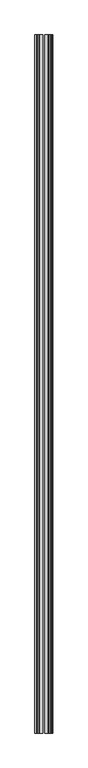
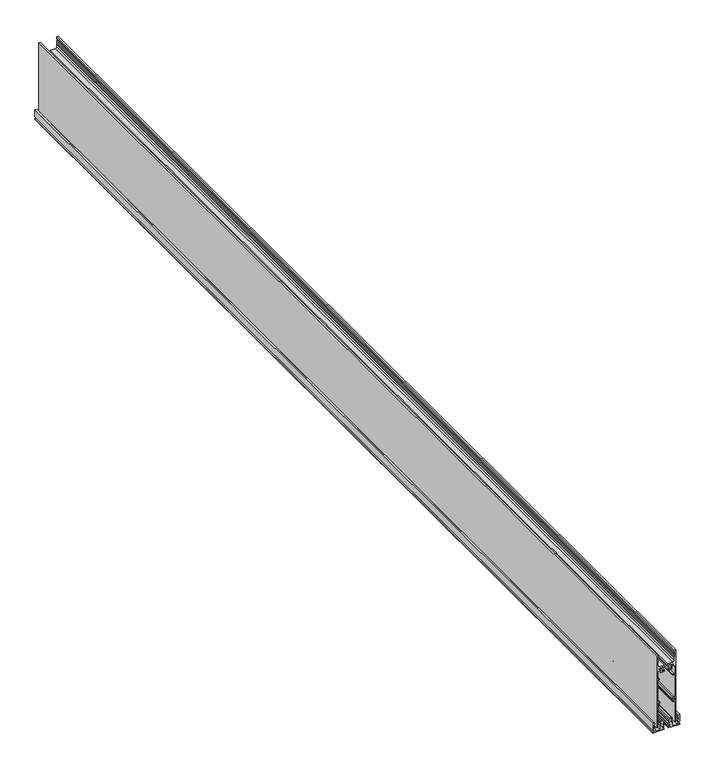
"""IFC4 building model written with IfcOpenShell, lengths in millimetres: proxy geometry, Structure002 653 : Structure002 653."""

from ifc_helpers import new_model, si_unit, frame, origin, place, context, project, spatial, polyline, outline, extrude, source, transform, mapped, element, save


def generic_models_8680b48e(model_context):
    return source(origin(), model_context, "Body", "SweptSolid", [
        extrude(outline(polyline([(37496.4365618, 7657.7930318), (37495.366697, 7656.7528175), (37493.1734209, 7656.7528175), (37493.1734209, 7657.8229747), (37494.7782571, 7657.8229747), (37494.7782571, 7659.1606712), (37486.7569596, 7659.1606712), (37486.7569596, 7657.8229747), (37488.3589123, 7657.8229747), (37488.3589123, 7656.7528175), (37485.0752597, 7656.7528175), (37483.4739937, 7655.8966918), (37479.1043438, 7655.8966918), (37479.1043438, 7646.8538638), (37488.3579135, 7646.8538638), (37488.3579135, 7645.7837066), (37486.7540761, 7645.7837066), (37486.7540761, 7644.4460101), (37494.7782571, 7644.4460101), (37494.7782571, 7645.7837066), (37493.1734209, 7645.7837066), (37493.1734209, 7646.8538638), (37495.366697, 7646.8538638), (37496.436721, 7645.7838398), (37496.436721, 7644.7135494), (37495.5512233, 7642.6415254), (37493.0931791, 7641.3693083), (37490.017243, 7641.3693083), (37490.017243, 7642.4394655), (37486.4063615, 7642.4394655), (37486.4063615, 7639.7636558), (37484.5340526, 7639.7636558), (37484.5340526, 7640.5671028), (37483.2789107, 7640.5671028), (37484.4508456, 7642.077477), (37484.4508456, 7643.199305), (37480.1257911, 7643.199305), (37479.7006783, 7643.9284483), (37479.2397502, 7643.1732751), (37479.2397502, 7641.7763334), (37480.6168771, 7641.7763334), (37480.6168771, 7640.2864915), (37479.8959721, 7639.724537), (37477.446, 7639.5315657), (37477.446, 7641.6449434), (37478.4679055, 7641.6449434), (37478.4679055, 7643.199305), (37477.446, 7643.199305), (37477.446, 7661.0334462), (37478.8903656, 7661.0334462), (37478.8903656, 7657.5554354), (37484.2874925, 7657.5554354), (37483.0336251, 7659.7088758), (37483.0336251, 7661.0334462), (37496.4365618, 7661.0334462), (37496.4365618, 7657.7930318)])), frame((0.0, -3747.9491938, 0.0), z_axis=(0.0, 1.0, 0.0), x_axis=(0.0, 0.0, 1.0)), (0.0, 0.0, 1.0), 2000.0),
        extrude(outline(polyline([(37483.0336251, 7610.0797736), (37483.0336251, 7611.404344), (37484.2874925, 7613.5577844), (37478.8903656, 7613.5577844), (37478.8903656, 7610.0797736), (37477.446, 7610.0797736), (37477.446, 7627.9139148), (37478.4679055, 7627.9139148), (37478.4679055, 7629.4682764), (37477.446, 7629.4682764), (37477.446, 7631.5816541), (37479.8959721, 7631.3886828), (37480.6168771, 7630.8267283), (37480.6168771, 7629.3368864), (37479.2397502, 7629.3368864), (37479.2397502, 7627.9399447), (37479.7006783, 7627.1847715), (37480.1257911, 7627.9139148), (37484.4508456, 7627.9139148), (37484.4508456, 7629.0357427), (37483.2789107, 7630.5461169), (37484.5340526, 7630.5461169), (37484.5340526, 7631.349564), (37486.4063615, 7631.349564), (37486.4063615, 7628.6737543), (37490.017243, 7628.6737543), (37490.017243, 7629.7439115), (37493.0931791, 7629.7439115), (37495.5512233, 7628.4716944), (37496.436721, 7626.3996703), (37496.436721, 7625.32938), (37495.366697, 7624.259356), (37493.1734209, 7624.259356), (37493.1734209, 7625.3295132), (37494.7782571, 7625.3295132), (37494.7782571, 7626.6672096), (37486.7540761, 7626.6672096), (37486.7540761, 7625.3295132), (37488.3579135, 7625.3295132), (37488.3579135, 7624.259356), (37479.1043438, 7624.259356), (37479.1043438, 7615.216528), (37483.4739937, 7615.216528), (37485.0752597, 7614.3604022), (37488.3589123, 7614.3604022), (37488.3589123, 7613.2902451), (37486.7569596, 7613.2902451), (37486.7569596, 7611.9525486), (37494.7782571, 7611.9525486), (37494.7782571, 7613.2902451), (37493.1734209, 7613.2902451), (37493.1734209, 7614.3604022), (37495.366697, 7614.3604022), (37496.4365618, 7613.320188), (37496.4365618, 7610.0797736), (37483.0336251, 7610.0797736)])), frame((0.0, -3747.9491938, 0.0), z_axis=(0.0, 1.0, 0.0), x_axis=(0.0, 0.0, 1.0)), (0.0, 0.0, 1.0), 2000.0),
        extrude(outline(polyline([(37604.2015618, 7622.5346434), (37606.7094313, 7620.0267738), (37611.5111794, 7620.0267738), (37613.3758754, 7620.5013448), (37616.0506024, 7619.6987269), (37616.0506024, 7620.5013448), (37618.7253294, 7619.6987269), (37618.7253294, 7620.5013448), (37621.4000564, 7619.6987269), (37621.4000564, 7620.5013448), (37624.0747835, 7619.6987269), (37624.0747835, 7620.5013448), (37626.7495105, 7620.5013448), (37626.7495105, 7617.5049047), (37485.4971771, 7617.5049047), (37485.4971771, 7620.019774), (37525.8320604, 7620.019774), (37525.8320604, 7622.9091984), (37527.4903911, 7622.9091984), (37527.4903911, 7621.9460569), (37529.4164343, 7620.0200138), (37532.9735815, 7620.0200138), (37532.9735815, 7621.8390412), (37531.2885035, 7621.8390412), (37531.2885035, 7623.444277), (37534.6319122, 7623.444277), (37534.6319122, 7620.019774), (37578.3369516, 7620.019774), (37578.3369516, 7622.9091984), (37579.9952823, 7622.9091984), (37579.9952823, 7620.019774), (37595.9502358, 7620.019774), (37595.9502358, 7620.9354673), (37597.8865057, 7622.2081155), (37599.3688896, 7621.4577733), (37600.7763445, 7621.4577733), (37601.7660928, 7623.391903), (37600.8580603, 7625.1625844), (37599.3688896, 7625.1625844), (37597.8866262, 7624.4666157), (37595.9502358, 7625.5845913), (37591.6838394, 7625.5845913), (37591.6838394, 7632.2730736), (37594.6795336, 7632.2730736), (37594.6795336, 7630.9353771), (37593.3421701, 7630.9353771), (37593.3421701, 7627.2433349), (37601.6873184, 7627.2433349), (37601.6873184, 7630.9353771), (37600.3499549, 7630.9353771), (37600.3499549, 7632.2730736), (37604.2015618, 7632.2730736), (37604.2015618, 7622.5346434)])), frame((0.0, -3747.9491938, 0.0), z_axis=(0.0, 1.0, 0.0), x_axis=(0.0, 0.0, 1.0)), (0.0, 0.0, 1.0), 2000.0),
        extrude(outline(polyline([(37600.3499549, 7638.8401462), (37600.3499549, 7640.1778427), (37601.6873184, 7640.1778427), (37601.6873184, 7643.8698849), (37593.3421701, 7643.8698849), (37593.3421701, 7640.1778427), (37594.6795336, 7640.1778427), (37594.6795336, 7638.8401462), (37591.6838394, 7638.8401462), (37591.6838394, 7645.5286285), (37595.9502358, 7645.5286285), (37597.8866262, 7646.646604), (37599.3688896, 7645.9506354), (37600.8580603, 7645.9506354), (37601.7660928, 7647.7213168), (37600.7763445, 7649.6554465), (37599.3688896, 7649.6554465), (37597.8865057, 7648.9051043), (37595.9502358, 7650.1777525), (37595.9502358, 7651.0934457), (37579.9952823, 7651.0934457), (37579.9952823, 7648.2040214), (37578.3369516, 7648.2040214), (37578.3369516, 7651.0934457), (37534.6319122, 7651.0934457), (37534.6319122, 7647.6689428), (37531.2885035, 7647.6689428), (37531.2885035, 7649.2741786), (37532.9735815, 7649.2741786), (37532.9735815, 7651.093206), (37529.4164343, 7651.093206), (37527.4903911, 7649.1671628), (37527.4903911, 7648.2040214), (37525.8320604, 7648.2040214), (37525.8320604, 7651.0934457), (37485.4971771, 7651.0934457), (37485.4971771, 7653.6083151), (37626.7495105, 7653.6083151), (37626.7495105, 7650.611875), (37624.0747835, 7650.611875), (37624.0747835, 7651.4144929), (37621.4000564, 7650.611875), (37621.4000564, 7651.4144929), (37618.7253294, 7650.611875), (37618.7253294, 7651.4144929), (37616.0506024, 7650.611875), (37616.0506024, 7651.4144929), (37613.3758754, 7650.611875), (37611.5111794, 7651.086446), (37606.7094313, 7651.086446), (37604.2015618, 7648.5785764), (37604.2015618, 7638.8401462), (37600.3499549, 7638.8401462)])), frame((0.0, -3747.9491938, 0.0), z_axis=(0.0, 1.0, 0.0), x_axis=(0.0, 0.0, 1.0)), (0.0, 0.0, 1.0), 2000.0),
    ])


if __name__ == "__main__":
    model = new_model("IFC4")
    model_context = context("Model", 3, world=origin())
    ifc_project = project(units=[si_unit("LENGTHUNIT", "METRE", prefix="MILLI")], contexts=[model_context])
    site = spatial("IfcSite", under=ifc_project)
    building = spatial("IfcBuilding", under=site)
    placement = place(None, origin())
    generic_models_shape = generic_models_8680b48e(model_context)
    element("IfcBuildingElementProxy", 1, Name="Structure002 653 : Structure002 653", ObjectType="Structure002 653 : Structure002 653", at=placement, inside=building, context=model_context, shape_type="MappedRepresentation", body=[
        mapped(generic_models_shape, transform((0.0, 0.0, 0.0), x_axis=(1.0, 0.0, 0.0), y_axis=(0.0, 1.0, 0.0), z_axis=(0.0, 0.0, 1.0))),
    ])
    save(model, "model.ifc")

# Revit data of these elements
# Type "Structure002 653 : Structure002 653"
#   NameOverride = "Structure002"
# Element 1 (IfcBuildingElementProxy, "Structure002 653 : Structure002 653")
#   Materials on its faces: "FLEETWOOD SLIDING DOOR SERIES 3070 (SEE ELEVATIONS FOR OPERABILITY)"
# Materials
#   "FLEETWOOD SLIDING DOOR SERIES 3070 (SEE ELEVATIONS FOR OPERABILITY)": class "Unassigned", colour RGB 143 136 136, transparency 0, Cost = 0
